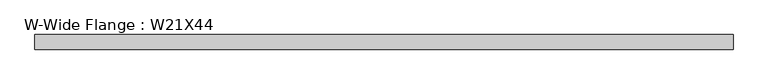
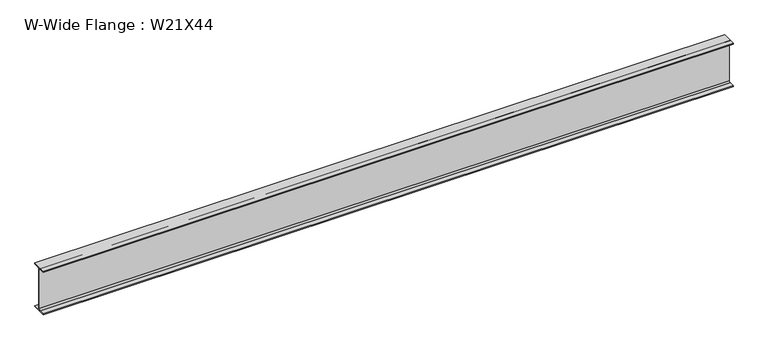
"""IFC4 building model written with IfcOpenShell, lengths in millimetres: beam geometry, W-Wide Flange : W21X44."""

from ifc_helpers import new_model, si_unit, point, frame, frame_2d, origin, place, context, project, spatial, polyline, circle_curve, trimmed, segment, composite_curve, outline, extrude, source, transform, mapped, element, save


def w_wide_flange_w21x44_476cda67(model_context):
    return source(origin(), model_context, "Body", "SweptSolid", [
        extrude(outline(composite_curve([segment(polyline([(82.55, -251.46), (82.55, -262.89), (-82.55, -262.89), (-82.55, -251.46), (-21.59, -251.46)]), True, "CONTINUOUS"), segment(trimmed(circle_curve(frame_2d((-21.59, -234.315)), 17.145), [point((-21.59, -251.46))], [point((-4.445, -234.315))], True, "CARTESIAN"), True, "CONTINUOUS"), segment(polyline([(-4.445, -234.315), (-4.445, 234.315)]), True, "CONTINUOUS"), segment(trimmed(circle_curve(frame_2d((-21.59, 234.315)), 17.145), [point((-4.445, 234.315))], [point((-21.59, 251.46))], True, "CARTESIAN"), True, "CONTINUOUS"), segment(polyline([(-21.59, 251.46), (-82.55, 251.46), (-82.55, 262.89), (82.55, 262.89), (82.55, 251.46), (21.59, 251.46)]), True, "CONTINUOUS"), segment(trimmed(circle_curve(frame_2d((21.59, 234.315)), 17.145), [point((21.59, 251.46))], [point((4.445, 234.315))], True, "CARTESIAN"), True, "CONTINUOUS"), segment(polyline([(4.445, 234.315), (4.445, -234.315)]), True, "CONTINUOUS"), segment(trimmed(circle_curve(frame_2d((21.59, -234.315)), 17.145), [point((4.445, -234.315))], [point((21.59, -251.46))], True, "CARTESIAN"), True, "CONTINUOUS"), segment(polyline([(21.59, -251.46), (82.55, -251.46)]), True, "CONTINUOUS")], self_intersect=False)), frame((-3902.8048239, 0.0, 0.0), z_axis=(1.0, 0.0, 0.0), x_axis=(0.0, 1.0, 0.0)), (0.0, 0.0, 1.0), 7866.3129601),
    ])


if __name__ == "__main__":
    model = new_model("IFC4")
    model_context = context("Model", 3, world=origin())
    ifc_project = project(units=[si_unit("LENGTHUNIT", "METRE", prefix="MILLI")], contexts=[model_context])
    site = spatial("IfcSite", under=ifc_project)
    building = spatial("IfcBuilding", under=site)
    placement = place(None, origin())
    w_wide_flange_w21x44_shape = w_wide_flange_w21x44_476cda67(model_context)
    element("IfcBeam", 1, ObjectType="W-Wide Flange : W21X44", at=placement, inside=building, context=model_context, shape_type="MappedRepresentation", body=[
        mapped(w_wide_flange_w21x44_shape, transform((0.0, 0.0, 0.0), x_axis=(1.0, 0.0, 0.0), y_axis=(0.0, 1.0, 0.0), z_axis=(0.0, 0.0, 1.0))),
    ])
    save(model, "model.ifc")

# Revit data of these elements
# Type "W-Wide Flange : W21X44"
#   Assembly Code = "B10"
#   W = 44
#   Length [instance default] = 1524 mm
#   bf = 165.1 mm
#   d = 525.78 mm
#   k = 28.575 mm
#   k2 = 17.145 mm
#   tf = 11.43 mm
#   tw = 8.89 mm
#   A = 0.00838708 m²
#   Structural Material [instance default] = Steel ASTM A992
# Element 1 (IfcBeam, "W-Wide Flange : W21X44")
#   Structural Material = Aluminum, Anodized Red
#   Materials on its faces: "Aluminum, Anodized Red"
# Materials
#   "Steel ASTM A992": class "Metal", colour RGB 128 0 0, transparency 0, Description = "Structural steel 50ksi", Cost = 0
#   "Aluminum, Anodized Red": class "Metal", colour RGB 120 120 120, transparency 0, Description = "Anodized aluminum, red", Cost = 0
